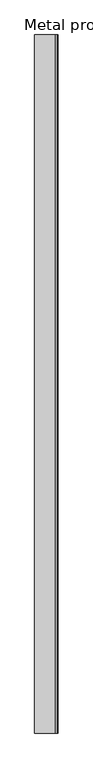
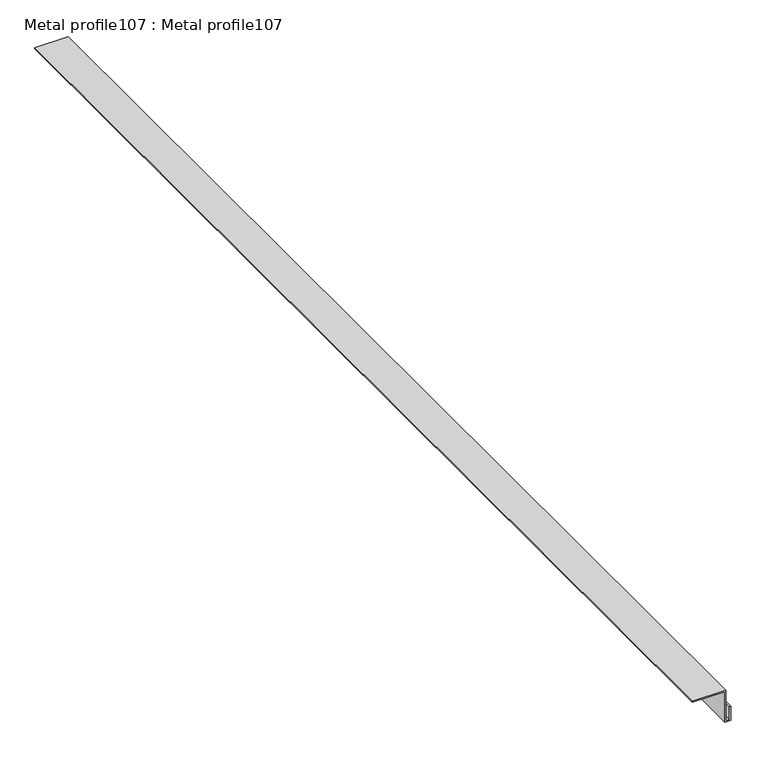
"""IFC4 building model written with IfcOpenShell, lengths in millimetres: proxy geometry, Metal profile107 : Metal profile107."""

from ifc_helpers import new_model, si_unit, frame, origin, place, context, project, spatial, polyline, outline, extrude, source, transform, mapped, element, save


def metal_profile107_metal_profile107_2f6635e2(model_context):
    return source(origin(), model_context, "Body", "SweptSolid", [
        extrude(outline(polyline([(41785.0836903, 6119.9286564), (41811.4586903, 6119.9286564), (41811.4586903, 6117.9286564), (41787.0836903, 6117.9286564), (41787.0836903, 6111.4652775), (41844.1930653, 6111.4652775), (41844.1930653, 6052.7890079), (41842.1930653, 6052.7890079), (41842.1930653, 6109.4652775), (41785.0836903, 6109.4652775), (41785.0836903, 6119.9286564)])), frame((0.0, 2217.3609988, 0.0), z_axis=(0.0, 1.0, 0.0), x_axis=(0.0, 0.0, 1.0)), (0.0, 0.0, 1.0), 2000.0),
    ])


if __name__ == "__main__":
    model = new_model("IFC4")
    model_context = context("Model", 3, world=origin())
    ifc_project = project(units=[si_unit("LENGTHUNIT", "METRE", prefix="MILLI")], contexts=[model_context])
    site = spatial("IfcSite", under=ifc_project)
    building = spatial("IfcBuilding", under=site)
    placement = place(None, origin())
    metal_profile107_metal_profile107_shape = metal_profile107_metal_profile107_2f6635e2(model_context)
    element("IfcBuildingElementProxy", 1, Name="Metal profile107 : Metal profile107", ObjectType="Metal profile107 : Metal profile107", at=placement, inside=building, context=model_context, shape_type="MappedRepresentation", body=[
        mapped(metal_profile107_metal_profile107_shape, transform((0.0, 0.0, 0.0), x_axis=(1.0, 0.0, 0.0), y_axis=(0.0, 1.0, 0.0), z_axis=(0.0, 0.0, 1.0))),
    ])
    save(model, "model.ifc")

# Revit data of these elements
# Type "Metal profile107 : Metal profile107"
#   NameOverride = "Metal profile107"
# Element 1 (IfcBuildingElementProxy, "Metal profile107 : Metal profile107")
#   Materials on its faces: "ANGLE TRIM"
# Materials
#   "ANGLE TRIM": class "Unassigned", colour RGB 245 226 176, transparency 0, Cost = 0
